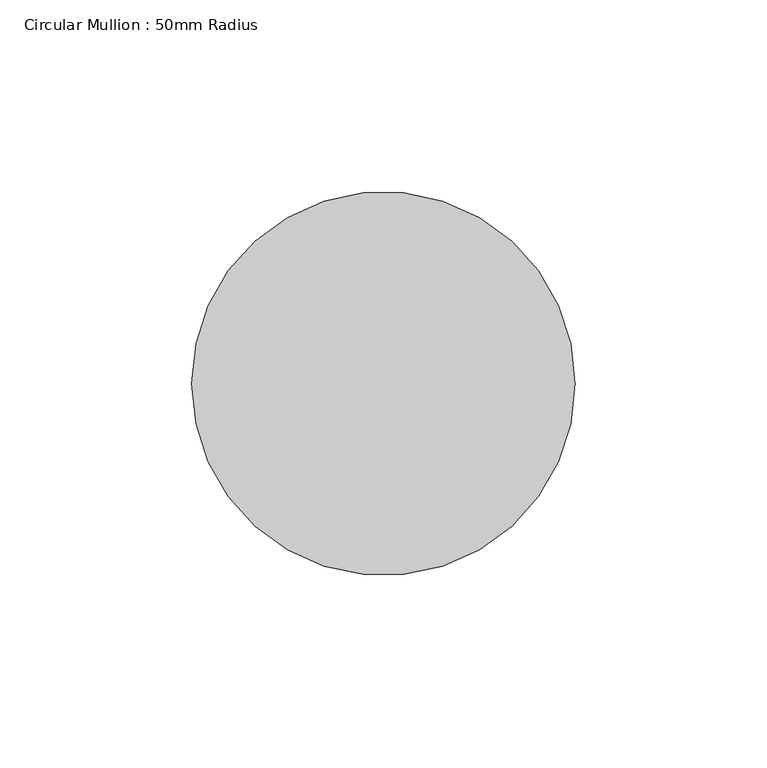
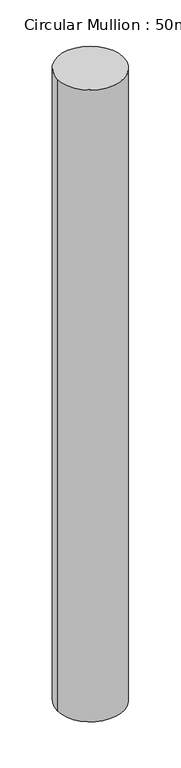
"""IFC4 building model written with IfcOpenShell, lengths in millimetres: member geometry, Circular Mullion : 50mm Radius."""

from ifc_helpers import new_model, si_unit, point, frame, origin, origin_2d, place, context, project, spatial, circle_curve, trimmed, segment, composite_curve, outline, extrude, source, transform, mapped, element, save


def circular_mullion_50mm_radius_2273e861(model_context):
    return source(origin(), model_context, "Body", "SweptSolid", [
        extrude(outline(composite_curve([segment(trimmed(circle_curve(origin_2d(), 50.0), [point((50.0, 0.0))], [point((-50.0, 0.0))], False, "CARTESIAN"), True, "CONTINUOUS"), segment(trimmed(circle_curve(origin_2d(), 50.0), [point((-50.0, 0.0))], [point((50.0, 0.0))], False, "CARTESIAN"), True, "CONTINUOUS")], self_intersect=False)), frame((0.0, 0.0, -1009.5976359), z_axis=(0.0, 0.0, 1.0), x_axis=(1.0, 0.0, 0.0)), (0.0, 0.0, 1.0), 1009.5976359),
    ])


if __name__ == "__main__":
    model = new_model("IFC4")
    model_context = context("Model", 3, world=origin())
    ifc_project = project(units=[si_unit("LENGTHUNIT", "METRE", prefix="MILLI")], contexts=[model_context])
    site = spatial("IfcSite", under=ifc_project)
    building = spatial("IfcBuilding", under=site)
    placement = place(None, origin())
    circular_mullion_50mm_radius_shape = circular_mullion_50mm_radius_2273e861(model_context)
    element("IfcMember", 1, ObjectType="Circular Mullion : 50mm Radius", at=placement, inside=building, context=model_context, shape_type="MappedRepresentation", body=[
        mapped(circular_mullion_50mm_radius_shape, transform((0.0, 0.0, 0.0), x_axis=(1.0, 0.0, 0.0), y_axis=(0.0, 1.0, 0.0), z_axis=(0.0, 0.0, 1.0))),
    ])
    save(model, "model.ifc")

# Revit data of these elements
# Type "Circular Mullion : 50mm Radius"
#   built-in parameter 1007350 = 0.164042 (stored number, unit not read)
# Element 1 (IfcMember, "Circular Mullion : 50mm Radius")
#   Materials on its faces: "Aluminium"
# Materials
#   "Aluminium": class "Metal", colour RGB 247 247 247, transparency 0, Description = "Aluminium 6061", Cost = 0
